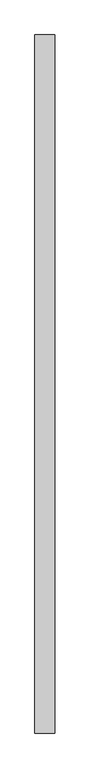
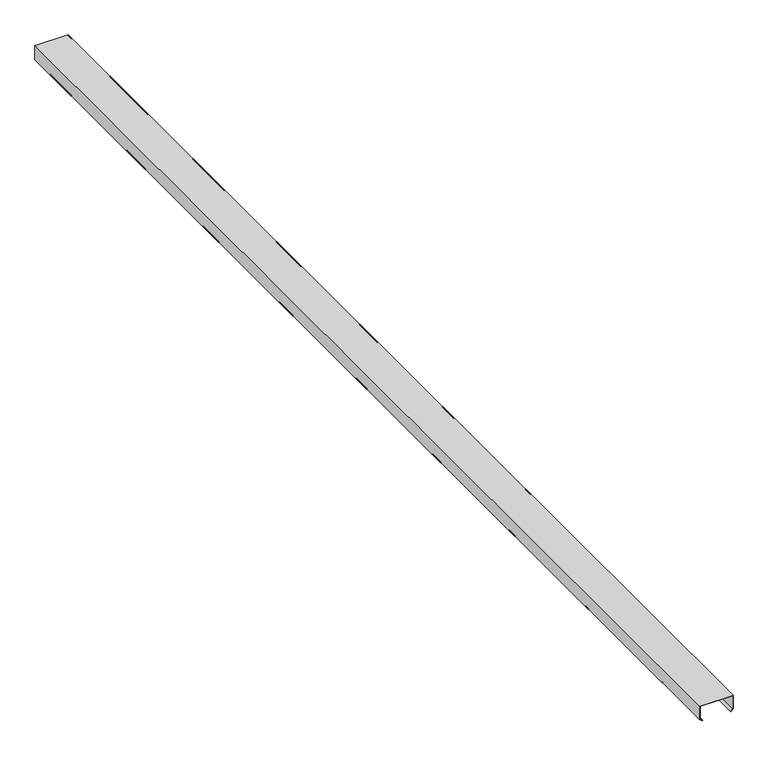
"""IFC4 building model written with IfcOpenShell, lengths in millimetres: proxy geometry, Generic Models 7:Generic Models 1:1:Generic Models 1:1 : Generic Models 7:Generic Models 1:337419:22 : Generic Models 7:Generic Models 1:1:Generic Models 1:1 : Generic Models 7:Generic Models 1:337419:306201."""

from ifc_helpers import new_model, si_unit, frame, origin, place, context, project, spatial, polyline, outline, extrude, source, transform, mapped, element, save


def generic_models_bf49e34b(model_context):
    return source(origin(), model_context, "Body", "SweptSolid", [
        extrude(outline(polyline([(4985.940625, 560556.1617239), (4985.940625, 560352.9617239), (4897.040625, 560352.9617239), (4884.7955211, 560367.5548705), (4886.9236883, 560369.3406148), (4898.336086, 560355.7398489), (4983.1625, 560355.7398489), (4983.1625, 560553.3835989), (4898.336086, 560553.3835989), (4886.9236883, 560539.7828329), (4884.7955211, 560541.5685772), (4897.040625, 560556.1617239), (4985.940625, 560556.1617239)])), frame((0.0, -578752.4153396, 0.0), z_axis=(0.0, 1.0, 0.0), x_axis=(0.0, 0.0, 1.0)), (0.0, 0.0, 1.0), 7066.9239556),
    ])


if __name__ == "__main__":
    model = new_model("IFC4")
    model_context = context("Model", 3, world=origin())
    ifc_project = project(units=[si_unit("LENGTHUNIT", "METRE", prefix="MILLI")], contexts=[model_context])
    site = spatial("IfcSite", under=ifc_project)
    building = spatial("IfcBuilding", under=site)
    placement = place(None, origin())
    generic_models_shape = generic_models_bf49e34b(model_context)
    element("IfcBuildingElementProxy", 1, Name="Generic Models 7:Generic Models 1:1:Generic Models 1:1 : Generic Models 7:Generic Models 1:337419:22 : Generic Models 7:Generic Models 1:1:Generic Models 1:1 : Generic Models 7:Generic Models 1:337419:306201", ObjectType="Generic Models 7:Generic Models 1:1:Generic Models 1:1 : Generic Models 7:Generic Models 1:337419:22 : Generic Models 7:Generic Models 1:1:Generic Models 1:1 : Generic Models 7:Generic Models 1:337419:306201", at=placement, inside=building, context=model_context, shape_type="MappedRepresentation", body=[
        mapped(generic_models_shape, transform((0.0, 0.0, 0.0), x_axis=(1.0, 0.0, 0.0), y_axis=(0.0, 1.0, 0.0), z_axis=(0.0, 0.0, 1.0))),
    ])
    save(model, "model.ifc")

# Revit data of these elements
# Type "Generic Models 7:Generic Models 1:1:Generic Models 1:1 : Generic Models 7:Generic Models 1:337419:22 : Generic Models 7:Generic Models 1:1:Generic Models 1:1 : Generic Models 7:Generic Models 1:337419:306201"
#   NameOverride = "Generic Models 7:Generic Models 1:1:Generic Models 1:1 : Generic Models 7:Generic Models 1:337419:306201"
#   ObjectTypeOverride = "Generic Models 1:1 : Generic Models 7:Generic Models 1:337419"
#   Reference = "Generic Models 1"
#   Tag = "306201"
# Element 1 (IfcBuildingElementProxy, "Generic Models 7:Generic Models 1:1:Generic Models 1:1 : Generic Models 7:Generic Models 1:337419:22 : Generic Models 7:Generic Models 1:1:Generic Models 1:1 : Generic Models 7:Generic Models 1:337419:306201")
#   Materials on its faces: "CEE' SECTION (8.0x3.5C - SEE STRUCT. DWGS)"
# Materials
#   "CEE' SECTION (8.0x3.5C - SEE STRUCT. DWGS)": class "Unassigned", colour RGB 210 209 208, transparency 0, Keynote = "M05121300.02", Cost = 0
